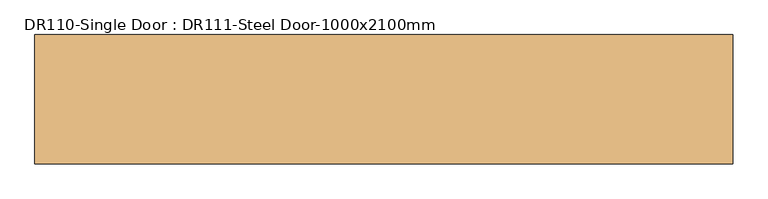
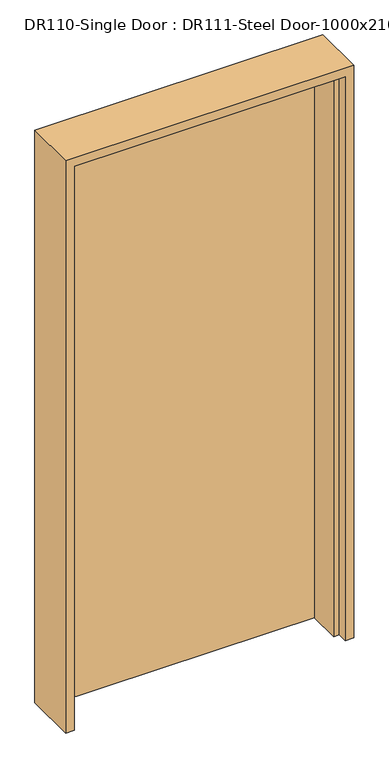
"""IFC4 building model written with IfcOpenShell, lengths in millimetres: door geometry, DR110-Single Door : DR111-Steel Door-1000x2100mm."""

from ifc_helpers import new_model, si_unit, origin, origin_with_axes, place, context, project, spatial, polyline, outline, extrude, faceted_brep, source, transform, mapped, element, save


def dr110_single_door_dr111_steel_door_1000x2100mm_0699664c(model_context):
    return source(origin(), model_context, "Body", "SolidModel", [
        extrude(outline(polyline([(470.0, 92.5), (470.0, 57.5), (-470.0, 57.5), (-470.0, 92.5), (470.0, 92.5)])), origin_with_axes(), (0.0, 0.0, 1.0), 2070.0),
        faceted_brep([(470.0, 92.5, 0.0), (500.0, 92.5, 0.0), (500.0, -92.5, 0.0), (470.0, -92.5, 0.0), (470.0, -57.5, 0.0), (450.0, -57.5, 0.0), (450.0, 57.5, 0.0), (470.0, 57.5, 0.0), (470.0, 92.5, 2070.0), (-470.0, 92.5, 2070.0), (-470.0, 92.5, 0.0), (-500.0, 92.5, 0.0), (-500.0, 92.5, 2100.0), (500.0, 92.5, 2100.0), (500.0, -92.5, 2100.0), (-500.0, -92.5, 2100.0), (-500.0, -92.5, 0.0), (-470.0, -92.5, 0.0), (-470.0, -92.5, 2070.0), (470.0, -92.5, 2070.0), (470.0, -57.5, 2070.0), (-470.0, -57.5, 2070.0), (-470.0, -57.5, 0.0), (-450.0, -57.5, 0.0), (-450.0, -57.5, 2050.0), (450.0, -57.5, 2050.0), (450.0, 57.5, 2050.0), (-450.0, 57.5, 2050.0), (-450.0, 57.5, 0.0), (-470.0, 57.5, 0.0), (-470.0, 57.5, 2070.0), (470.0, 57.5, 2070.0)], [[[0, 1, 2, 3, 4, 5, 6, 7]], [[1, 0, 8, 9, 10, 11, 12, 13]], [[2, 1, 13, 14]], [[3, 2, 14, 15, 16, 17, 18, 19]], [[4, 3, 19, 20]], [[5, 4, 20, 21, 22, 23, 24, 25]], [[6, 5, 25, 26]], [[7, 6, 26, 27, 28, 29, 30, 31]], [[0, 7, 31, 8]], [[9, 30, 29, 10]], [[10, 29, 28, 23, 22, 17, 16, 11]], [[15, 12, 11, 16]], [[21, 18, 17, 22]], [[27, 24, 23, 28]], [[14, 13, 12, 15]], [[20, 19, 18, 21]], [[26, 25, 24, 27]], [[8, 31, 30, 9]]]),
    ])


if __name__ == "__main__":
    model = new_model("IFC4")
    model_context = context("Model", 3, world=origin())
    ifc_project = project(units=[si_unit("LENGTHUNIT", "METRE", prefix="MILLI")], contexts=[model_context])
    site = spatial("IfcSite", under=ifc_project)
    building = spatial("IfcBuilding", under=site)
    placement = place(None, origin())
    dr110_single_door_dr111_steel_door_1000x2100mm_shape = dr110_single_door_dr111_steel_door_1000x2100mm_0699664c(model_context)
    element("IfcDoor", 1, ObjectType="DR110-Single Door : DR111-Steel Door-1000x2100mm", at=placement, inside=building, context=model_context, shape_type="MappedRepresentation", body=[
        mapped(dr110_single_door_dr111_steel_door_1000x2100mm_shape, transform((0.0, 0.0, 0.0), x_axis=(1.0, 0.0, 0.0), y_axis=(0.0, 1.0, 0.0), z_axis=(0.0, 0.0, 1.0))),
    ])
    save(model, "model.ifc")

# Revit data of these elements
# Type "DR110-Single Door : DR111-Steel Door-1000x2100mm"
#   Description = "DSDSSD"
#   Type Mark = "SD"
#   Analytic Construction = "<None>"
#   프레임 투영 외부. = 25 mm
#   프레임 투영 내부. = 25 mm
#   프레임 폭 = 75 mm
#   Height = 2100 mm
#   Width = 1000 mm
#   Define Thermal Properties by = 1
#   문 패널 = SD1 문 패널
#   문 프레임 = A04AQ098-00002_Steel Door_non FP_single
#   Function = (empty or 0)
#   Wall Closure = (empty or 0)
# Element 1 (IfcDoor, "DR110-Single Door : DR111-Steel Door-1000x2100mm")
#   Materials on its faces: "A04AQ098-00002_Steel Door_non FP_single", "SD1 문 패널"
# Materials
#   "SD1 문 패널": class "금속", colour RGB 247 247 247, transparency 0, Description = "STEEL DOOR (1000Wx2100H)"
#   "A04AQ098-00002_Steel Door_non FP_single": class "금속", colour RGB 247 247 247, transparency 0, Description = "Steel Door", W00) Work Master Code = "A04AQ098-00002", W01) Work Master_Lv1 = "Finishing Work", W02) Work Master_Lv2 = "Door & Window Work", W03) Work Master_Spec.1 = "Steel Door w/ Steel Frame", W04) Work Master_Spec.2 = "Fire Protective Rating: N/A, Single Door", W05) Work Master_Spec.3 = "w/ Hardware & Accessories", Cost = 0
